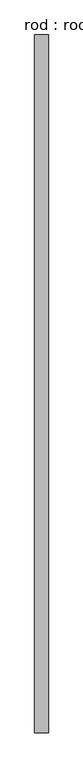
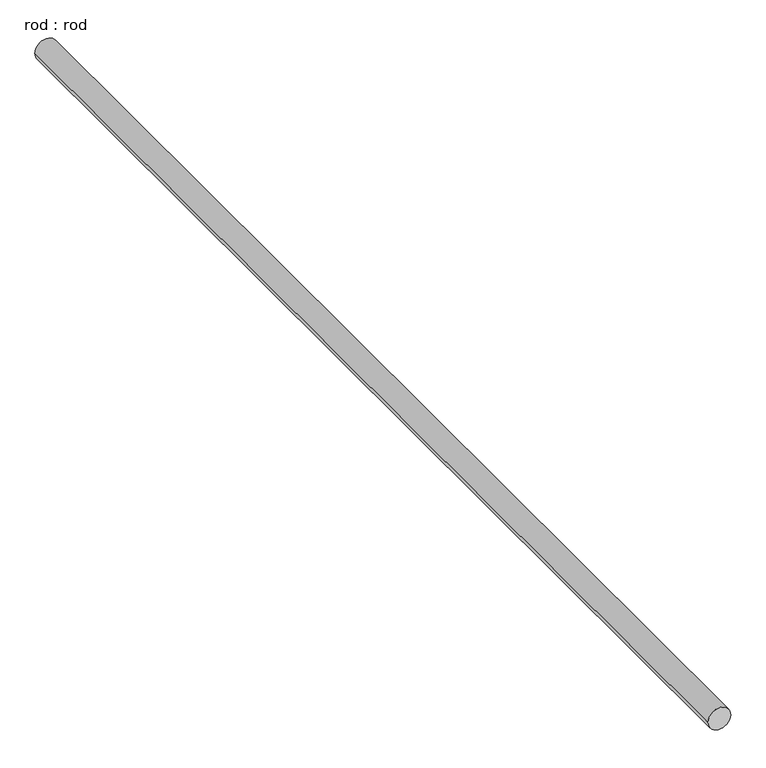
"""IFC4 building model written with IfcOpenShell, lengths in millimetres: proxy geometry, rod : rod."""

import ifcopenshell
import ifcopenshell.guid

model = None  # the IFC model being written
_history = None  # IfcOwnerHistory: only IFC2X3 demands one
_inside = {}  # id of a spatial element -> (the spatial element, [elements in it])
_under = {}  # id of a project, library or spatial element -> (it, [spatial elements below it])
_declared = {}  # id of a project -> (the project, [libraries it declares])
_typed = {}  # id of a type object -> (the type object, [elements of that type])
_made_of = {}  # id of a material, layer set ... -> (it, [elements and type objects made of it])


def new_model(schema):
    """Start an empty IFC model of exactly this schema.

    Asked for "IFC4X3", IfcOpenShell would pick the latest addendum, in which some entities
    have other attributes; the version numbers below select the first issue.
    IFC2X3 requires an IfcOwnerHistory on every rooted entity: one is made here for all.
    """
    global model, _history
    if schema == "IFC4X3":
        model = ifcopenshell.file(schema_version=(4, 3, 0, 0))
    else:
        model = ifcopenshell.file(schema=schema)
    _inside.clear()
    _under.clear()
    _declared.clear()
    _typed.clear()
    _made_of.clear()
    _history = None
    if model.schema == "IFC2X3":
        org = make("IfcOrganization", Name="unknown")
        user = make(
            "IfcPersonAndOrganization",
            ThePerson=make("IfcPerson", FamilyName="unknown"),
            TheOrganization=org,
        )
        app = make(
            "IfcApplication",
            ApplicationDeveloper=org,
            Version="unknown",
            ApplicationFullName="unknown",
            ApplicationIdentifier="unknown",
        )
        _history = make(
            "IfcOwnerHistory",
            OwningUser=user,
            OwningApplication=app,
            ChangeAction="ADDED",
            CreationDate=0,
        )
    return model


def make(cls, **values):
    """One entity of the class cls with the attributes given. An attribute that is None is left unset."""
    return model.create_entity(
        cls, **{name: value for name, value in values.items() if value is not None}
    )


def rooted(cls, **values):
    """An entity with a GlobalId (a new one), such as an element, a storey or a relation."""
    return make(cls, GlobalId=ifcopenshell.guid.new(), OwnerHistory=_history, **values)


def si_unit(unit_type, name, prefix=None):
    """IfcSIUnit, for example si_unit("LENGTHUNIT", "METRE", prefix="MILLI")."""
    return make("IfcSIUnit", UnitType=unit_type, Prefix=prefix, Name=name)


def assignment(units):
    """IfcUnitAssignment: the units of a project."""
    return None if units is None else make("IfcUnitAssignment", Units=units)


def point(xyz):
    """IfcCartesianPoint."""
    return None if xyz is None else make("IfcCartesianPoint", Coordinates=xyz)


def direction(xyz):
    """IfcDirection."""
    return None if xyz is None else make("IfcDirection", DirectionRatios=xyz)


def frame(location, z_axis=None, x_axis=None):
    """IfcAxis2Placement3D, a coordinate frame: its origin and axes. An axis left out is left unset."""
    return make(
        "IfcAxis2Placement3D",
        Location=point(location),
        Axis=direction(z_axis),
        RefDirection=direction(x_axis),
    )


def frame_2d(location, x_axis=None):
    """IfcAxis2Placement2D, a coordinate frame in the plane: its origin and x axis."""
    return make(
        "IfcAxis2Placement2D", Location=point(location), RefDirection=direction(x_axis)
    )


def origin():
    """The frame at (0, 0, 0) with its axes left unset."""
    return frame((0.0, 0.0, 0.0))


def place(relative_to, where):
    """IfcLocalPlacement: puts the frame where relative to a parent placement (None: the world)."""
    return make(
        "IfcLocalPlacement", PlacementRelTo=relative_to, RelativePlacement=where
    )


def context(
    kind, dimensions, precision=None, world=None, true_north=None, identifier=None
):
    """IfcGeometricRepresentationContext, for example the 3D "Model" context."""
    return make(
        "IfcGeometricRepresentationContext",
        ContextIdentifier=identifier,
        ContextType=kind,
        CoordinateSpaceDimension=dimensions,
        Precision=precision,
        WorldCoordinateSystem=world,
        TrueNorth=true_north,
    )


def project(units=None, contexts=None):
    """IfcProject with its units and contexts."""
    return rooted(
        "IfcProject",
        Name="project",
        RepresentationContexts=contexts,
        UnitsInContext=assignment(units),
    )


def spatial(cls, under=None, at=None, **own):
    """A site, building, storey or space (cls), placed at a placement, below another one or the project."""
    s = rooted(cls, ObjectPlacement=at, **own)
    if under is not None:
        _under.setdefault(under.id(), (under, []))[1].append(s)
    return s


def circle_curve(where, radius):
    """IfcCircle in the frame where."""
    return make("IfcCircle", Position=where, Radius=radius)


def trimmed(basis, trim1, trim2, sense, master):
    """IfcTrimmedCurve: the piece of a basis curve between two trims."""
    return make(
        "IfcTrimmedCurve",
        BasisCurve=basis,
        Trim1=trim1,
        Trim2=trim2,
        SenseAgreement=sense,
        MasterRepresentation=master,
    )


def segment(curve, same_sense, transition):
    """IfcCompositeCurveSegment."""
    return make(
        "IfcCompositeCurveSegment",
        Transition=transition,
        SameSense=same_sense,
        ParentCurve=curve,
    )


def composite_curve(segments, self_intersect=None):
    """IfcCompositeCurve: segments joined end to end."""
    return make("IfcCompositeCurve", Segments=segments, SelfIntersect=self_intersect)


def outline(outer, holes=None, kind="AREA"):
    """IfcArbitraryClosedProfileDef: a profile drawn as a closed curve; with holes, ...WithVoids."""
    if holes is None:
        return make("IfcArbitraryClosedProfileDef", ProfileType=kind, OuterCurve=outer)
    return make(
        "IfcArbitraryProfileDefWithVoids",
        ProfileType=kind,
        OuterCurve=outer,
        InnerCurves=holes,
    )


def extrude(swept, where, along, depth):
    """IfcExtrudedAreaSolid: the profile swept, set in the frame where, extruded along a direction by depth."""
    return make(
        "IfcExtrudedAreaSolid",
        SweptArea=swept,
        Position=where,
        ExtrudedDirection=direction(along),
        Depth=depth,
    )


def shape(context_of_items, identifier, shape_type, items):
    """IfcShapeRepresentation: the items that make up one representation, for example the "Body"."""
    return make(
        "IfcShapeRepresentation",
        ContextOfItems=context_of_items,
        RepresentationIdentifier=identifier,
        RepresentationType=shape_type,
        Items=items,
    )


def source(mapping_origin, context_of_items, identifier, shape_type, items):
    """IfcRepresentationMap: a shape defined once, which mapped items show again and again."""
    return make(
        "IfcRepresentationMap",
        MappingOrigin=mapping_origin,
        MappedRepresentation=shape(context_of_items, identifier, shape_type, items),
    )


def transform(
    local_origin,
    x_axis=None,
    y_axis=None,
    z_axis=None,
    scale=None,
    scale2=None,
    scale3=None,
    uniform=True,
):
    """IfcCartesianTransformationOperator3D, or its non-uniform kind. x_axis, y_axis, z_axis: its Axis1, 2, 3."""
    if uniform:
        return make(
            "IfcCartesianTransformationOperator3D",
            Axis1=direction(x_axis),
            Axis2=direction(y_axis),
            LocalOrigin=point(local_origin),
            Scale=scale,
            Axis3=direction(z_axis),
        )
    return make(
        "IfcCartesianTransformationOperator3DnonUniform",
        Axis1=direction(x_axis),
        Axis2=direction(y_axis),
        LocalOrigin=point(local_origin),
        Scale=scale,
        Axis3=direction(z_axis),
        Scale2=scale2,
        Scale3=scale3,
    )


def mapped(mapping_source, mapping_target):
    """IfcMappedItem: shows the shape of a source again, moved by a transform."""
    return make(
        "IfcMappedItem", MappingSource=mapping_source, MappingTarget=mapping_target
    )


def made_of(thing, what):
    """Note that an element or type object is made of a material, layer set ...; save() writes the relation."""
    if what is not None:
        _made_of.setdefault(what.id(), (what, []))[1].append(thing)
    return thing


def element(
    cls,
    number,
    at=None,
    inside=None,
    cuts=None,
    type_object=None,
    material=None,
    context=None,
    identifier="Body",
    shape_type=None,
    held_by="IfcProductDefinitionShape",
    body=None,
    shapes=None,
    **own,
):
    """One element of the class cls, such as IfcWall. Its Tag is "e" and its number.

    at: its placement. inside: the storey or other place that contains it. cuts: it is an
    opening in that element (IfcRelVoidsElement). A single representation is given by context,
    identifier, shape_type and body (its items); several are given by shapes. held_by: the class
    of the entity that holds the representations. save() writes the other relations.
    """
    e = rooted(cls, Tag="e%d" % number, ObjectPlacement=at, **own)
    if body is not None:
        shapes = [shape(context, identifier, shape_type, body)]
    if shapes is not None:
        e.Representation = make(held_by, Representations=shapes)
    if inside is not None:
        _inside.setdefault(inside.id(), (inside, []))[1].append(e)
    if cuts is not None:
        rooted(
            "IfcRelVoidsElement", RelatingBuildingElement=cuts, RelatedOpeningElement=e
        )
    if type_object is not None:
        _typed.setdefault(type_object.id(), (type_object, []))[1].append(e)
    return made_of(e, material)


def aggregate(whole, parts):
    """IfcRelAggregates: a whole, such as a stair, and the parts it consists of."""
    return rooted("IfcRelAggregates", RelatingObject=whole, RelatedObjects=parts)


def save(model, path):
    """Write the relations noted so far, then the file.

    IfcRelAggregates (storeys below a building ...), IfcRelContainedInSpatialStructure (elements
    in a storey), IfcRelDefinesByType, IfcRelAssociatesMaterial and IfcRelDeclares: one each for
    every whole, place, type object, material and project.
    """
    for whole, parts in _under.values():
        aggregate(whole, parts)
    for where, things in _inside.values():
        rooted(
            "IfcRelContainedInSpatialStructure",
            RelatedElements=things,
            RelatingStructure=where,
        )
    for kind, things in _typed.values():
        rooted("IfcRelDefinesByType", RelatedObjects=things, RelatingType=kind)
    for what, things in _made_of.values():
        rooted("IfcRelAssociatesMaterial", RelatedObjects=things, RelatingMaterial=what)
    for by, libraries in _declared.values():
        rooted("IfcRelDeclares", RelatingContext=by, RelatedDefinitions=libraries)
    model.write(path)


def rod_rod_e610b66d(model_context):
    return source(origin(), model_context, "Body", "SweptSolid", [
        extrude(outline(composite_curve([segment(trimmed(circle_curve(frame_2d((0.0108462, 0.0)), 200.0), [point((0.0108462, 200.0))], [point((0.0108462, -200.0))], False, "CARTESIAN"), True, "CONTINUOUS"), segment(trimmed(circle_curve(frame_2d((0.0108462, 0.0)), 200.0), [point((0.0108462, -200.0))], [point((0.0108462, 200.0))], False, "CARTESIAN"), True, "CONTINUOUS")], self_intersect=False)), frame((0.0, -6139.4142418, 0.0), z_axis=(0.0, 1.0, 0.0), x_axis=(0.0, 0.0, 1.0)), (0.0, 0.0, 1.0), 20464.2857143),
    ])


if __name__ == "__main__":
    model = new_model("IFC4")
    model_context = context("Model", 3, world=origin())
    ifc_project = project(units=[si_unit("LENGTHUNIT", "METRE", prefix="MILLI")], contexts=[model_context])
    site = spatial("IfcSite", under=ifc_project)
    building = spatial("IfcBuilding", under=site)
    placement = place(None, origin())
    rod_rod_shape = rod_rod_e610b66d(model_context)
    element("IfcBuildingElementProxy", 1, Name="rod : rod", ObjectType="rod : rod", at=placement, inside=building, context=model_context, shape_type="MappedRepresentation", body=[
        mapped(rod_rod_shape, transform((0.0, 0.0, 0.0), x_axis=(1.0, 0.0, 0.0), y_axis=(0.0, 1.0, 0.0), z_axis=(0.0, 0.0, 1.0))),
    ])
    save(model, "model.ifc")

# Revit data of these elements
# Type "rod : rod"
#   Default Elevation = 0
